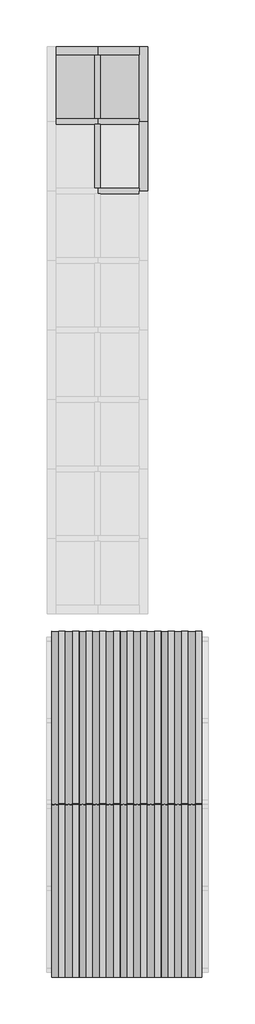
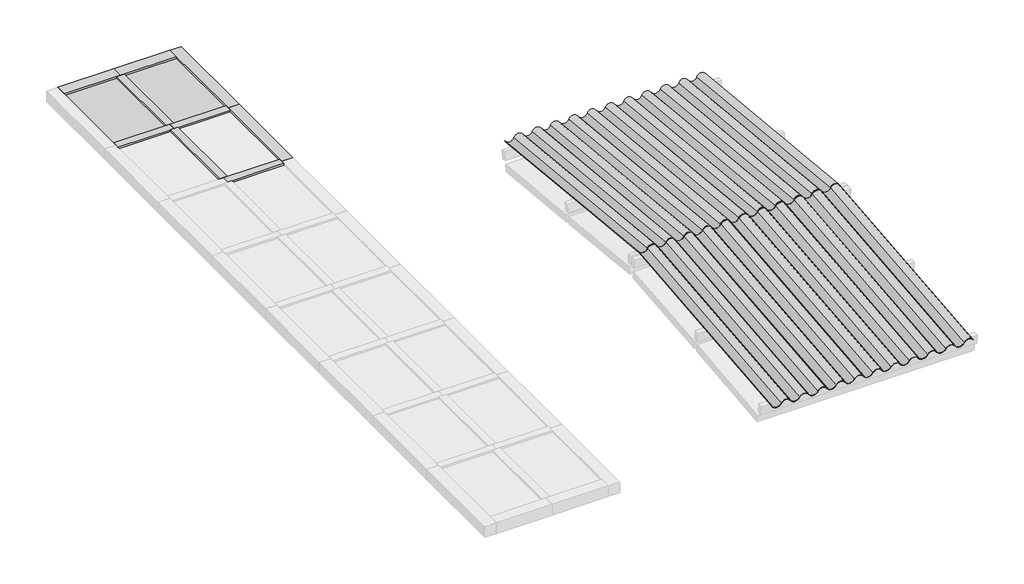
# One storey, part 2 of 2: 22 beams, 9 members, 2 plates.
"""IFC4 building model written with IfcOpenShell, lengths in millimetres."""

import ifcopenshell
import ifcopenshell.guid

model = None  # the IFC model being written
_history = None  # IfcOwnerHistory: only IFC2X3 demands one
_inside = {}  # id of a spatial element -> (the spatial element, [elements in it])
_under = {}  # id of a project, library or spatial element -> (it, [spatial elements below it])
_declared = {}  # id of a project -> (the project, [libraries it declares])
_typed = {}  # id of a type object -> (the type object, [elements of that type])
_made_of = {}  # id of a material, layer set ... -> (it, [elements and type objects made of it])


def new_model(schema):
    """Start an empty IFC model of exactly this schema.

    Asked for "IFC4X3", IfcOpenShell would pick the latest addendum, in which some entities
    have other attributes; the version numbers below select the first issue.
    IFC2X3 requires an IfcOwnerHistory on every rooted entity: one is made here for all.
    """
    global model, _history
    if schema == "IFC4X3":
        model = ifcopenshell.file(schema_version=(4, 3, 0, 0))
    else:
        model = ifcopenshell.file(schema=schema)
    _inside.clear()
    _under.clear()
    _declared.clear()
    _typed.clear()
    _made_of.clear()
    _history = None
    if model.schema == "IFC2X3":
        org = make("IfcOrganization", Name="unknown")
        user = make(
            "IfcPersonAndOrganization",
            ThePerson=make("IfcPerson", FamilyName="unknown"),
            TheOrganization=org,
        )
        app = make(
            "IfcApplication",
            ApplicationDeveloper=org,
            Version="unknown",
            ApplicationFullName="unknown",
            ApplicationIdentifier="unknown",
        )
        _history = make(
            "IfcOwnerHistory",
            OwningUser=user,
            OwningApplication=app,
            ChangeAction="ADDED",
            CreationDate=0,
        )
    return model


def make(cls, **values):
    """One entity of the class cls with the attributes given. An attribute that is None is left unset."""
    return model.create_entity(
        cls, **{name: value for name, value in values.items() if value is not None}
    )


def rooted(cls, **values):
    """An entity with a GlobalId (a new one), such as an element, a storey or a relation."""
    return make(cls, GlobalId=ifcopenshell.guid.new(), OwnerHistory=_history, **values)


def si_unit(unit_type, name, prefix=None):
    """IfcSIUnit, for example si_unit("LENGTHUNIT", "METRE", prefix="MILLI")."""
    return make("IfcSIUnit", UnitType=unit_type, Prefix=prefix, Name=name)


def assignment(units):
    """IfcUnitAssignment: the units of a project."""
    return None if units is None else make("IfcUnitAssignment", Units=units)


def point(xyz):
    """IfcCartesianPoint."""
    return None if xyz is None else make("IfcCartesianPoint", Coordinates=xyz)


def direction(xyz):
    """IfcDirection."""
    return None if xyz is None else make("IfcDirection", DirectionRatios=xyz)


def frame(location, z_axis=None, x_axis=None):
    """IfcAxis2Placement3D, a coordinate frame: its origin and axes. An axis left out is left unset."""
    return make(
        "IfcAxis2Placement3D",
        Location=point(location),
        Axis=direction(z_axis),
        RefDirection=direction(x_axis),
    )


def frame_2d(location, x_axis=None):
    """IfcAxis2Placement2D, a coordinate frame in the plane: its origin and x axis."""
    return make(
        "IfcAxis2Placement2D", Location=point(location), RefDirection=direction(x_axis)
    )


def origin():
    """The frame at (0, 0, 0) with its axes left unset."""
    return frame((0.0, 0.0, 0.0))


def origin_with_axes():
    """The frame at (0, 0, 0) with the z axis (0, 0, 1) and the x axis (1, 0, 0) written out."""
    return frame((0.0, 0.0, 0.0), z_axis=(0.0, 0.0, 1.0), x_axis=(1.0, 0.0, 0.0))


def place(relative_to, where):
    """IfcLocalPlacement: puts the frame where relative to a parent placement (None: the world)."""
    return make(
        "IfcLocalPlacement", PlacementRelTo=relative_to, RelativePlacement=where
    )


def context(
    kind, dimensions, precision=None, world=None, true_north=None, identifier=None
):
    """IfcGeometricRepresentationContext, for example the 3D "Model" context."""
    return make(
        "IfcGeometricRepresentationContext",
        ContextIdentifier=identifier,
        ContextType=kind,
        CoordinateSpaceDimension=dimensions,
        Precision=precision,
        WorldCoordinateSystem=world,
        TrueNorth=true_north,
    )


def project(units=None, contexts=None):
    """IfcProject with its units and contexts."""
    return rooted(
        "IfcProject",
        Name="project",
        RepresentationContexts=contexts,
        UnitsInContext=assignment(units),
    )


def spatial(cls, under=None, at=None, **own):
    """A site, building, storey or space (cls), placed at a placement, below another one or the project."""
    s = rooted(cls, ObjectPlacement=at, **own)
    if under is not None:
        _under.setdefault(under.id(), (under, []))[1].append(s)
    return s


def polyline(points):
    """IfcPolyline through the points."""
    return make("IfcPolyline", Points=[point(p) for p in points])


def circle_curve(where, radius):
    """IfcCircle in the frame where."""
    return make("IfcCircle", Position=where, Radius=radius)


def trimmed(basis, trim1, trim2, sense, master):
    """IfcTrimmedCurve: the piece of a basis curve between two trims."""
    return make(
        "IfcTrimmedCurve",
        BasisCurve=basis,
        Trim1=trim1,
        Trim2=trim2,
        SenseAgreement=sense,
        MasterRepresentation=master,
    )


def segment(curve, same_sense, transition):
    """IfcCompositeCurveSegment."""
    return make(
        "IfcCompositeCurveSegment",
        Transition=transition,
        SameSense=same_sense,
        ParentCurve=curve,
    )


def composite_curve(segments, self_intersect=None):
    """IfcCompositeCurve: segments joined end to end."""
    return make("IfcCompositeCurve", Segments=segments, SelfIntersect=self_intersect)


def outline(outer, holes=None, kind="AREA"):
    """IfcArbitraryClosedProfileDef: a profile drawn as a closed curve; with holes, ...WithVoids."""
    if holes is None:
        return make("IfcArbitraryClosedProfileDef", ProfileType=kind, OuterCurve=outer)
    return make(
        "IfcArbitraryProfileDefWithVoids",
        ProfileType=kind,
        OuterCurve=outer,
        InnerCurves=holes,
    )


def extrude(swept, where, along, depth):
    """IfcExtrudedAreaSolid: the profile swept, set in the frame where, extruded along a direction by depth."""
    return make(
        "IfcExtrudedAreaSolid",
        SweptArea=swept,
        Position=where,
        ExtrudedDirection=direction(along),
        Depth=depth,
    )


def shape(context_of_items, identifier, shape_type, items):
    """IfcShapeRepresentation: the items that make up one representation, for example the "Body"."""
    return make(
        "IfcShapeRepresentation",
        ContextOfItems=context_of_items,
        RepresentationIdentifier=identifier,
        RepresentationType=shape_type,
        Items=items,
    )


def source(mapping_origin, context_of_items, identifier, shape_type, items):
    """IfcRepresentationMap: a shape defined once, which mapped items show again and again."""
    return make(
        "IfcRepresentationMap",
        MappingOrigin=mapping_origin,
        MappedRepresentation=shape(context_of_items, identifier, shape_type, items),
    )


def transform(
    local_origin,
    x_axis=None,
    y_axis=None,
    z_axis=None,
    scale=None,
    scale2=None,
    scale3=None,
    uniform=True,
):
    """IfcCartesianTransformationOperator3D, or its non-uniform kind. x_axis, y_axis, z_axis: its Axis1, 2, 3."""
    if uniform:
        return make(
            "IfcCartesianTransformationOperator3D",
            Axis1=direction(x_axis),
            Axis2=direction(y_axis),
            LocalOrigin=point(local_origin),
            Scale=scale,
            Axis3=direction(z_axis),
        )
    return make(
        "IfcCartesianTransformationOperator3DnonUniform",
        Axis1=direction(x_axis),
        Axis2=direction(y_axis),
        LocalOrigin=point(local_origin),
        Scale=scale,
        Axis3=direction(z_axis),
        Scale2=scale2,
        Scale3=scale3,
    )


def mapped(mapping_source, mapping_target):
    """IfcMappedItem: shows the shape of a source again, moved by a transform."""
    return make(
        "IfcMappedItem", MappingSource=mapping_source, MappingTarget=mapping_target
    )


def made_of(thing, what):
    """Note that an element or type object is made of a material, layer set ...; save() writes the relation."""
    if what is not None:
        _made_of.setdefault(what.id(), (what, []))[1].append(thing)
    return thing


def element(
    cls,
    number,
    at=None,
    inside=None,
    cuts=None,
    type_object=None,
    material=None,
    context=None,
    identifier="Body",
    shape_type=None,
    held_by="IfcProductDefinitionShape",
    body=None,
    shapes=None,
    **own,
):
    """One element of the class cls, such as IfcWall. Its Tag is "e" and its number.

    at: its placement. inside: the storey or other place that contains it. cuts: it is an
    opening in that element (IfcRelVoidsElement). A single representation is given by context,
    identifier, shape_type and body (its items); several are given by shapes. held_by: the class
    of the entity that holds the representations. save() writes the other relations.
    """
    e = rooted(cls, Tag="e%d" % number, ObjectPlacement=at, **own)
    if body is not None:
        shapes = [shape(context, identifier, shape_type, body)]
    if shapes is not None:
        e.Representation = make(held_by, Representations=shapes)
    if inside is not None:
        _inside.setdefault(inside.id(), (inside, []))[1].append(e)
    if cuts is not None:
        rooted(
            "IfcRelVoidsElement", RelatingBuildingElement=cuts, RelatedOpeningElement=e
        )
    if type_object is not None:
        _typed.setdefault(type_object.id(), (type_object, []))[1].append(e)
    return made_of(e, material)


def aggregate(whole, parts):
    """IfcRelAggregates: a whole, such as a stair, and the parts it consists of."""
    return rooted("IfcRelAggregates", RelatingObject=whole, RelatedObjects=parts)


def save(model, path):
    """Write the relations noted so far, then the file.

    IfcRelAggregates (storeys below a building ...), IfcRelContainedInSpatialStructure (elements
    in a storey), IfcRelDefinesByType, IfcRelAssociatesMaterial and IfcRelDeclares: one each for
    every whole, place, type object, material and project.
    """
    for whole, parts in _under.values():
        aggregate(whole, parts)
    for where, things in _inside.values():
        rooted(
            "IfcRelContainedInSpatialStructure",
            RelatedElements=things,
            RelatingStructure=where,
        )
    for kind, things in _typed.values():
        rooted("IfcRelDefinesByType", RelatedObjects=things, RelatingType=kind)
    for what, things in _made_of.values():
        rooted("IfcRelAssociatesMaterial", RelatedObjects=things, RelatingMaterial=what)
    for by, libraries in _declared.values():
        rooted("IfcRelDeclares", RelatingContext=by, RelatedDefinitions=libraries)
    model.write(path)


def montante_retangular_d0ec09bd(model_context):
    return source(origin(), model_context, "Body", "SweptSolid", [
        extrude(outline(polyline([(50.0, 75.0), (50.0, -75.0), (-50.0, -75.0), (-50.0, 75.0), (50.0, 75.0)])), frame((0.0, 0.0, -1143.7500002), z_axis=(0.0, 0.0, 1.0), x_axis=(1.0, 0.0, 0.0)), (0.0, 0.0, 1.0), 1143.7500002),
    ])


def montante_retangular_ab766952(model_context):
    return source(origin(), model_context, "Body", "SweptSolid", [
        extrude(outline(polyline([(50.0, 75.0), (50.0, -75.0), (-50.0, -75.0), (-50.0, 75.0), (50.0, 75.0)])), frame((0.0, 0.0, -750.0), z_axis=(0.0, 0.0, 1.0), x_axis=(1.0, 0.0, 0.0)), (0.0, 0.0, 1.0), 750.0),
    ])


def montante_retangular_cc_150_x_150_mm_106b3bff(model_context):
    return source(origin(), model_context, "Body", "SweptSolid", [
        extrude(outline(polyline([(0.0, 75.0), (0.0, -75.0), (-150.0, -75.0), (-150.0, 75.0), (0.0, 75.0)])), frame((0.0, 0.0, -1343.7500002), z_axis=(0.0, 0.0, 1.0), x_axis=(1.0, 0.0, 0.0)), (0.0, 0.0, 1.0), 1343.7500002),
    ])


def montante_retangular_cc_150_x_150_mm_9af7129c(model_context):
    return source(origin(), model_context, "Body", "SweptSolid", [
        extrude(outline(polyline([(0.0, 75.0), (0.0, -75.0), (-150.0, -75.0), (-150.0, 75.0), (0.0, 75.0)])), frame((0.0, 0.0, -750.0), z_axis=(0.0, 0.0, 1.0), x_axis=(1.0, 0.0, 0.0)), (0.0, 0.0, 1.0), 750.0),
    ])


def montante_retangular_cc_150_x_150_mm_95775847(model_context):
    return source(origin(), model_context, "Body", "SweptSolid", [
        extrude(outline(polyline([(0.0, 75.0), (0.0, -75.0), (-150.0, -75.0), (-150.0, 75.0), (0.0, 75.0)])), frame((0.0, 0.0, -1243.7499999), z_axis=(0.0, 0.0, 1.0), x_axis=(1.0, 0.0, 0.0)), (0.0, 0.0, 1.0), 1243.7499999),
    ])


def painel_do_sistema_e7d0d29a(model_context):
    return source(origin(), model_context, "Body", "SweptSolid", [
        extrude(outline(polyline([(571.8750001, -49.5), (-571.8750001, -49.5), (-571.8750001, -24.5), (571.8750001, -24.5), (571.8750001, -49.5)])), origin_with_axes(), (0.0, 0.0, 1.0), 700.0),
    ])


model = new_model("IFC4")

# Units and contexts
model_context = context("Model", 3, world=origin())
ifc_project = project(units=[si_unit("LENGTHUNIT", "METRE", prefix="MILLI")], contexts=[model_context])

# Site, building, storey
site = spatial("IfcSite", under=ifc_project)
building = spatial("IfcBuilding", under=site)
storey = spatial("IfcBuildingStorey", under=building, Name="COB. CAIXA D'ÁGUA", Elevation=8750.0)

# Beams
placement = place(None, origin())
element("IfcBeam", 1, ObjectType="Telha Ondulada : Fibrocimento", at=placement, inside=storey, context=model_context, shape_type="SweptSolid", body=[
    extrude(outline(composite_curve([segment(trimmed(circle_curve(frame_2d((-58.7002978, -53.2060539)), 66.7939461), [point((-29.3501489, 6.7939461))], [point((-29.3501489, -113.2060539))], False, "CARTESIAN"), True, "CONTINUOUS"), segment(polyline([(-29.3501489, -113.2060539), (-31.5472154, -108.7146289)]), True, "CONTINUOUS"), segment(trimmed(circle_curve(frame_2d((-58.7002978, -53.2060539)), 61.7939461), [point((-31.5472154, -108.7146289))], [point((-31.5472154, 2.3025211))], True, "CARTESIAN"), True, "CONTINUOUS"), segment(trimmed(circle_curve(frame_2d((0.0, 66.7939461)), 71.7939461), [point((-31.5472154, 2.3025211))], [point((-31.5472154, 131.2853711))], False, "CARTESIAN"), True, "CONTINUOUS"), segment(polyline([(-31.5472154, 131.2853711), (-29.3501489, 126.7939461)]), True, "CONTINUOUS"), segment(trimmed(circle_curve(frame_2d((0.0, 66.7939461)), 66.7939461), [point((-29.3501489, 126.7939461))], [point((-29.3501489, 6.7939461))], True, "CARTESIAN"), True, "CONTINUOUS")], self_intersect=False)), frame((199.6156257, -4662.1614585, 9090.9296777), z_axis=(0.0, -0.9950371902099893, 0.09950371902099821), x_axis=(0.0, 0.09950371902099821, 0.9950371902099893)), (0.0, 0.0, 1.0), 3103.677649),
])
element("IfcBeam", 2, ObjectType="Telha Ondulada : Fibrocimento", at=placement, inside=storey, context=model_context, shape_type="SweptSolid", body=[
    extrude(outline(composite_curve([segment(trimmed(circle_curve(frame_2d((-58.7002978, -53.2060539)), 66.7939461), [point((-29.3501489, 6.7939461))], [point((-29.3501489, -113.2060539))], False, "CARTESIAN"), True, "CONTINUOUS"), segment(polyline([(-29.3501489, -113.2060539), (-31.5472154, -108.7146289)]), True, "CONTINUOUS"), segment(trimmed(circle_curve(frame_2d((-58.7002978, -53.2060539)), 61.7939461), [point((-31.5472154, -108.7146289))], [point((-31.5472154, 2.3025211))], True, "CARTESIAN"), True, "CONTINUOUS"), segment(trimmed(circle_curve(frame_2d((0.0, 66.7939461)), 71.7939461), [point((-31.5472154, 2.3025211))], [point((-31.5472154, 131.2853711))], False, "CARTESIAN"), True, "CONTINUOUS"), segment(polyline([(-31.5472154, 131.2853711), (-29.3501489, 126.7939461)]), True, "CONTINUOUS"), segment(trimmed(circle_curve(frame_2d((0.0, 66.7939461)), 66.7939461), [point((-29.3501489, 126.7939461))], [point((-29.3501489, 6.7939461))], True, "CARTESIAN"), True, "CONTINUOUS")], self_intersect=False)), frame((444.1156257, -4662.1614585, 9090.9296777), z_axis=(0.0, -0.9950371902099893, 0.09950371902099821), x_axis=(0.0, 0.09950371902099821, 0.9950371902099893)), (0.0, 0.0, 1.0), 3103.677649),
])
element("IfcBeam", 3, ObjectType="Telha Ondulada : Fibrocimento", at=placement, inside=storey, context=model_context, shape_type="SweptSolid", body=[
    extrude(outline(composite_curve([segment(trimmed(circle_curve(frame_2d((-58.7002978, -53.2060539)), 66.7939461), [point((-29.3501489, 6.7939461))], [point((-29.3501489, -113.2060539))], False, "CARTESIAN"), True, "CONTINUOUS"), segment(polyline([(-29.3501489, -113.2060539), (-31.5472154, -108.7146289)]), True, "CONTINUOUS"), segment(trimmed(circle_curve(frame_2d((-58.7002978, -53.2060539)), 61.7939461), [point((-31.5472154, -108.7146289))], [point((-31.5472154, 2.3025211))], True, "CARTESIAN"), True, "CONTINUOUS"), segment(trimmed(circle_curve(frame_2d((0.0, 66.7939461)), 71.7939461), [point((-31.5472154, 2.3025211))], [point((-31.5472154, 131.2853711))], False, "CARTESIAN"), True, "CONTINUOUS"), segment(polyline([(-31.5472154, 131.2853711), (-29.3501489, 126.7939461)]), True, "CONTINUOUS"), segment(trimmed(circle_curve(frame_2d((0.0, 66.7939461)), 66.7939461), [point((-29.3501489, 126.7939461))], [point((-29.3501489, 6.7939461))], True, "CARTESIAN"), True, "CONTINUOUS")], self_intersect=False)), frame((688.6156257, -4662.1614585, 9090.9296777), z_axis=(0.0, -0.9950371902099893, 0.09950371902099821), x_axis=(0.0, 0.09950371902099821, 0.9950371902099893)), (0.0, 0.0, 1.0), 3103.677649),
])
element("IfcBeam", 4, ObjectType="Telha Ondulada : Fibrocimento", at=placement, inside=storey, context=model_context, shape_type="SweptSolid", body=[
    extrude(outline(composite_curve([segment(trimmed(circle_curve(frame_2d((-58.7002978, -53.2060539)), 66.7939461), [point((-29.3501489, 6.7939461))], [point((-29.3501489, -113.2060539))], False, "CARTESIAN"), True, "CONTINUOUS"), segment(polyline([(-29.3501489, -113.2060539), (-31.5472154, -108.7146289)]), True, "CONTINUOUS"), segment(trimmed(circle_curve(frame_2d((-58.7002978, -53.2060539)), 61.7939461), [point((-31.5472154, -108.7146289))], [point((-31.5472154, 2.3025211))], True, "CARTESIAN"), True, "CONTINUOUS"), segment(trimmed(circle_curve(frame_2d((0.0, 66.7939461)), 71.7939461), [point((-31.5472154, 2.3025211))], [point((-31.5472154, 131.2853711))], False, "CARTESIAN"), True, "CONTINUOUS"), segment(polyline([(-31.5472154, 131.2853711), (-29.3501489, 126.7939461)]), True, "CONTINUOUS"), segment(trimmed(circle_curve(frame_2d((0.0, 66.7939461)), 66.7939461), [point((-29.3501489, 126.7939461))], [point((-29.3501489, 6.7939461))], True, "CARTESIAN"), True, "CONTINUOUS")], self_intersect=False)), frame((933.1156257, -4662.1614585, 9090.9296777), z_axis=(0.0, -0.9950371902099893, 0.09950371902099821), x_axis=(0.0, 0.09950371902099821, 0.9950371902099893)), (0.0, 0.0, 1.0), 3103.677649),
])
element("IfcBeam", 5, ObjectType="Telha Ondulada : Fibrocimento", at=placement, inside=storey, context=model_context, shape_type="SweptSolid", body=[
    extrude(outline(composite_curve([segment(trimmed(circle_curve(frame_2d((-58.7002978, -53.2060539)), 66.7939461), [point((-29.3501489, 6.7939461))], [point((-29.3501489, -113.2060539))], False, "CARTESIAN"), True, "CONTINUOUS"), segment(polyline([(-29.3501489, -113.2060539), (-31.5472154, -108.7146289)]), True, "CONTINUOUS"), segment(trimmed(circle_curve(frame_2d((-58.7002978, -53.2060539)), 61.7939461), [point((-31.5472154, -108.7146289))], [point((-31.5472154, 2.3025211))], True, "CARTESIAN"), True, "CONTINUOUS"), segment(trimmed(circle_curve(frame_2d((0.0, 66.7939461)), 71.7939461), [point((-31.5472154, 2.3025211))], [point((-31.5472154, 131.2853711))], False, "CARTESIAN"), True, "CONTINUOUS"), segment(polyline([(-31.5472154, 131.2853711), (-29.3501489, 126.7939461)]), True, "CONTINUOUS"), segment(trimmed(circle_curve(frame_2d((0.0, 66.7939461)), 66.7939461), [point((-29.3501489, 126.7939461))], [point((-29.3501489, 6.7939461))], True, "CARTESIAN"), True, "CONTINUOUS")], self_intersect=False)), frame((1177.6156257, -4662.1614585, 9090.9296777), z_axis=(0.0, -0.9950371902099893, 0.09950371902099821), x_axis=(0.0, 0.09950371902099821, 0.9950371902099893)), (0.0, 0.0, 1.0), 3103.677649),
])
element("IfcBeam", 6, ObjectType="Telha Ondulada : Fibrocimento", at=placement, inside=storey, context=model_context, shape_type="SweptSolid", body=[
    extrude(outline(composite_curve([segment(trimmed(circle_curve(frame_2d((-58.7002978, -53.2060539)), 66.7939461), [point((-29.3501489, 6.7939461))], [point((-29.3501489, -113.2060539))], False, "CARTESIAN"), True, "CONTINUOUS"), segment(polyline([(-29.3501489, -113.2060539), (-31.5472154, -108.7146289)]), True, "CONTINUOUS"), segment(trimmed(circle_curve(frame_2d((-58.7002978, -53.2060539)), 61.7939461), [point((-31.5472154, -108.7146289))], [point((-31.5472154, 2.3025211))], True, "CARTESIAN"), True, "CONTINUOUS"), segment(trimmed(circle_curve(frame_2d((0.0, 66.7939461)), 71.7939461), [point((-31.5472154, 2.3025211))], [point((-31.5472154, 131.2853711))], False, "CARTESIAN"), True, "CONTINUOUS"), segment(polyline([(-31.5472154, 131.2853711), (-29.3501489, 126.7939461)]), True, "CONTINUOUS"), segment(trimmed(circle_curve(frame_2d((0.0, 66.7939461)), 66.7939461), [point((-29.3501489, 126.7939461))], [point((-29.3501489, 6.7939461))], True, "CARTESIAN"), True, "CONTINUOUS")], self_intersect=False)), frame((1422.1156257, -4662.1614585, 9090.9296777), z_axis=(0.0, -0.9950371902099893, 0.09950371902099789), x_axis=(0.0, 0.09950371902099789, 0.9950371902099893)), (0.0, 0.0, 1.0), 3103.677649),
])
element("IfcBeam", 7, ObjectType="Telha Ondulada : Fibrocimento", at=placement, inside=storey, context=model_context, shape_type="SweptSolid", body=[
    extrude(outline(composite_curve([segment(trimmed(circle_curve(frame_2d((-58.7002978, -53.2060539)), 66.7939461), [point((-29.3501489, 6.7939461))], [point((-29.3501489, -113.2060539))], False, "CARTESIAN"), True, "CONTINUOUS"), segment(polyline([(-29.3501489, -113.2060539), (-31.5472154, -108.7146289)]), True, "CONTINUOUS"), segment(trimmed(circle_curve(frame_2d((-58.7002978, -53.2060539)), 61.7939461), [point((-31.5472154, -108.7146289))], [point((-31.5472154, 2.3025211))], True, "CARTESIAN"), True, "CONTINUOUS"), segment(trimmed(circle_curve(frame_2d((0.0, 66.7939461)), 71.7939461), [point((-31.5472154, 2.3025211))], [point((-31.5472154, 131.2853711))], False, "CARTESIAN"), True, "CONTINUOUS"), segment(polyline([(-31.5472154, 131.2853711), (-29.3501489, 126.7939461)]), True, "CONTINUOUS"), segment(trimmed(circle_curve(frame_2d((0.0, 66.7939461)), 66.7939461), [point((-29.3501489, 126.7939461))], [point((-29.3501489, 6.7939461))], True, "CARTESIAN"), True, "CONTINUOUS")], self_intersect=False)), frame((1666.6156257, -4662.1614585, 9090.9296777), z_axis=(0.0, -0.9950371902099893, 0.09950371902099789), x_axis=(0.0, 0.09950371902099789, 0.9950371902099893)), (0.0, 0.0, 1.0), 3103.677649),
])
element("IfcBeam", 8, ObjectType="Telha Ondulada : Fibrocimento", at=placement, inside=storey, context=model_context, shape_type="SweptSolid", body=[
    extrude(outline(composite_curve([segment(trimmed(circle_curve(frame_2d((-58.7002978, -53.2060539)), 66.7939461), [point((-29.3501489, 6.7939461))], [point((-29.3501489, -113.2060539))], False, "CARTESIAN"), True, "CONTINUOUS"), segment(polyline([(-29.3501489, -113.2060539), (-31.5472154, -108.7146289)]), True, "CONTINUOUS"), segment(trimmed(circle_curve(frame_2d((-58.7002978, -53.2060539)), 61.7939461), [point((-31.5472154, -108.7146289))], [point((-31.5472154, 2.3025211))], True, "CARTESIAN"), True, "CONTINUOUS"), segment(trimmed(circle_curve(frame_2d((0.0, 66.7939461)), 71.7939461), [point((-31.5472154, 2.3025211))], [point((-31.5472154, 131.2853711))], False, "CARTESIAN"), True, "CONTINUOUS"), segment(polyline([(-31.5472154, 131.2853711), (-29.3501489, 126.7939461)]), True, "CONTINUOUS"), segment(trimmed(circle_curve(frame_2d((0.0, 66.7939461)), 66.7939461), [point((-29.3501489, 126.7939461))], [point((-29.3501489, 6.7939461))], True, "CARTESIAN"), True, "CONTINUOUS")], self_intersect=False)), frame((1911.1156257, -4662.1614585, 9090.9296777), z_axis=(0.0, -0.9950371902099893, 0.09950371902099789), x_axis=(0.0, 0.09950371902099789, 0.9950371902099893)), (0.0, 0.0, 1.0), 3103.677649),
])
element("IfcBeam", 9, ObjectType="Telha Ondulada : Fibrocimento", at=placement, inside=storey, context=model_context, shape_type="SweptSolid", body=[
    extrude(outline(composite_curve([segment(trimmed(circle_curve(frame_2d((-58.7002978, -53.2060539)), 66.7939461), [point((-29.3501489, 6.7939461))], [point((-29.3501489, -113.2060539))], False, "CARTESIAN"), True, "CONTINUOUS"), segment(polyline([(-29.3501489, -113.2060539), (-31.5472154, -108.7146289)]), True, "CONTINUOUS"), segment(trimmed(circle_curve(frame_2d((-58.7002978, -53.2060539)), 61.7939461), [point((-31.5472154, -108.7146289))], [point((-31.5472154, 2.3025211))], True, "CARTESIAN"), True, "CONTINUOUS"), segment(trimmed(circle_curve(frame_2d((0.0, 66.7939461)), 71.7939461), [point((-31.5472154, 2.3025211))], [point((-31.5472154, 131.2853711))], False, "CARTESIAN"), True, "CONTINUOUS"), segment(polyline([(-31.5472154, 131.2853711), (-29.3501489, 126.7939461)]), True, "CONTINUOUS"), segment(trimmed(circle_curve(frame_2d((0.0, 66.7939461)), 66.7939461), [point((-29.3501489, 126.7939461))], [point((-29.3501489, 6.7939461))], True, "CARTESIAN"), True, "CONTINUOUS")], self_intersect=False)), frame((2155.6156257, -4662.1614585, 9090.9296777), z_axis=(0.0, -0.9950371902099893, 0.09950371902099789), x_axis=(0.0, 0.09950371902099789, 0.9950371902099893)), (0.0, 0.0, 1.0), 3103.677649),
])
element("IfcBeam", 10, ObjectType="Telha Ondulada : Fibrocimento", at=placement, inside=storey, context=model_context, shape_type="SweptSolid", body=[
    extrude(outline(composite_curve([segment(trimmed(circle_curve(frame_2d((-58.7002978, -53.2060539)), 66.7939461), [point((-29.3501489, 6.7939461))], [point((-29.3501489, -113.2060539))], False, "CARTESIAN"), True, "CONTINUOUS"), segment(polyline([(-29.3501489, -113.2060539), (-31.5472154, -108.7146289)]), True, "CONTINUOUS"), segment(trimmed(circle_curve(frame_2d((-58.7002978, -53.2060539)), 61.7939461), [point((-31.5472154, -108.7146289))], [point((-31.5472154, 2.3025211))], True, "CARTESIAN"), True, "CONTINUOUS"), segment(trimmed(circle_curve(frame_2d((0.0, 66.7939461)), 71.7939461), [point((-31.5472154, 2.3025211))], [point((-31.5472154, 131.2853711))], False, "CARTESIAN"), True, "CONTINUOUS"), segment(polyline([(-31.5472154, 131.2853711), (-29.3501489, 126.7939461)]), True, "CONTINUOUS"), segment(trimmed(circle_curve(frame_2d((0.0, 66.7939461)), 66.7939461), [point((-29.3501489, 126.7939461))], [point((-29.3501489, 6.7939461))], True, "CARTESIAN"), True, "CONTINUOUS")], self_intersect=False)), frame((2400.1156257, -4662.1614585, 9090.9296777), z_axis=(0.0, -0.9950371902099893, 0.09950371902099789), x_axis=(0.0, 0.09950371902099789, 0.9950371902099893)), (0.0, 0.0, 1.0), 3103.677649),
])
element("IfcBeam", 11, ObjectType="Telha Ondulada : Fibrocimento", at=placement, inside=storey, context=model_context, shape_type="SweptSolid", body=[
    extrude(outline(composite_curve([segment(trimmed(circle_curve(frame_2d((-58.7002978, -53.2060539)), 66.7939461), [point((-29.3501489, 6.7939461))], [point((-29.3501489, -113.2060539))], False, "CARTESIAN"), True, "CONTINUOUS"), segment(polyline([(-29.3501489, -113.2060539), (-31.5472154, -108.7146289)]), True, "CONTINUOUS"), segment(trimmed(circle_curve(frame_2d((-58.7002978, -53.2060539)), 61.7939461), [point((-31.5472154, -108.7146289))], [point((-31.5472154, 2.3025211))], True, "CARTESIAN"), True, "CONTINUOUS"), segment(trimmed(circle_curve(frame_2d((0.0, 66.7939461)), 71.7939461), [point((-31.5472154, 2.3025211))], [point((-31.5472154, 131.2853711))], False, "CARTESIAN"), True, "CONTINUOUS"), segment(polyline([(-31.5472154, 131.2853711), (-29.3501489, 126.7939461)]), True, "CONTINUOUS"), segment(trimmed(circle_curve(frame_2d((0.0, 66.7939461)), 66.7939461), [point((-29.3501489, 126.7939461))], [point((-29.3501489, 6.7939461))], True, "CARTESIAN"), True, "CONTINUOUS")], self_intersect=False)), frame((2644.6156257, -4662.1614585, 9090.9296777), z_axis=(0.0, -0.9950371902099893, 0.09950371902099789), x_axis=(0.0, 0.09950371902099789, 0.9950371902099893)), (0.0, 0.0, 1.0), 3103.677649),
])
element("IfcBeam", 12, ObjectType="Telha Ondulada : Fibrocimento", at=placement, inside=storey, context=model_context, shape_type="SweptSolid", body=[
    extrude(outline(composite_curve([segment(trimmed(circle_curve(frame_2d((0.0, 66.7939461)), 66.7939461), [point((29.3501489, 6.7939461))], [point((29.3501489, 126.7939461))], True, "CARTESIAN"), True, "CONTINUOUS"), segment(polyline([(29.3501489, 126.7939461), (31.5472154, 131.2853711)]), True, "CONTINUOUS"), segment(trimmed(circle_curve(frame_2d((0.0, 66.7939461)), 71.7939461), [point((31.5472154, 131.2853711))], [point((31.5472154, 2.3025211))], False, "CARTESIAN"), True, "CONTINUOUS"), segment(trimmed(circle_curve(frame_2d((58.7002978, -53.2060539)), 61.7939461), [point((31.5472154, 2.3025211))], [point((31.5472154, -108.7146289))], True, "CARTESIAN"), True, "CONTINUOUS"), segment(polyline([(31.5472154, -108.7146289), (29.3501489, -113.2060539)]), True, "CONTINUOUS"), segment(trimmed(circle_curve(frame_2d((58.7002978, -53.2060539)), 66.7939461), [point((29.3501489, -113.2060539))], [point((29.3501489, 6.7939461))], False, "CARTESIAN"), True, "CONTINUOUS")], self_intersect=False)), frame((199.6156257, -10856.9785109, 9090.7496777), z_axis=(0.0, 0.9950371902099894, 0.09950371902099744), x_axis=(0.0, 0.09950371902099744, -0.9950371902099894)), (0.0, 0.0, 1.0), 3103.677649),
])
element("IfcBeam", 13, ObjectType="Telha Ondulada : Fibrocimento", at=placement, inside=storey, context=model_context, shape_type="SweptSolid", body=[
    extrude(outline(composite_curve([segment(trimmed(circle_curve(frame_2d((0.0, 66.7939461)), 66.7939461), [point((29.3501489, 6.7939461))], [point((29.3501489, 126.7939461))], True, "CARTESIAN"), True, "CONTINUOUS"), segment(polyline([(29.3501489, 126.7939461), (31.5472154, 131.2853711)]), True, "CONTINUOUS"), segment(trimmed(circle_curve(frame_2d((0.0, 66.7939461)), 71.7939461), [point((31.5472154, 131.2853711))], [point((31.5472154, 2.3025211))], False, "CARTESIAN"), True, "CONTINUOUS"), segment(trimmed(circle_curve(frame_2d((58.7002978, -53.2060539)), 61.7939461), [point((31.5472154, 2.3025211))], [point((31.5472154, -108.7146289))], True, "CARTESIAN"), True, "CONTINUOUS"), segment(polyline([(31.5472154, -108.7146289), (29.3501489, -113.2060539)]), True, "CONTINUOUS"), segment(trimmed(circle_curve(frame_2d((58.7002978, -53.2060539)), 66.7939461), [point((29.3501489, -113.2060539))], [point((29.3501489, 6.7939461))], False, "CARTESIAN"), True, "CONTINUOUS")], self_intersect=False)), frame((444.1156257, -10856.9785109, 9090.7496777), z_axis=(0.0, 0.9950371902099894, 0.09950371902099744), x_axis=(0.0, 0.09950371902099744, -0.9950371902099894)), (0.0, 0.0, 1.0), 3103.677649),
])
element("IfcBeam", 14, ObjectType="Telha Ondulada : Fibrocimento", at=placement, inside=storey, context=model_context, shape_type="SweptSolid", body=[
    extrude(outline(composite_curve([segment(trimmed(circle_curve(frame_2d((0.0, 66.7939461)), 66.7939461), [point((29.3501489, 6.7939461))], [point((29.3501489, 126.7939461))], True, "CARTESIAN"), True, "CONTINUOUS"), segment(polyline([(29.3501489, 126.7939461), (31.5472154, 131.2853711)]), True, "CONTINUOUS"), segment(trimmed(circle_curve(frame_2d((0.0, 66.7939461)), 71.7939461), [point((31.5472154, 131.2853711))], [point((31.5472154, 2.3025211))], False, "CARTESIAN"), True, "CONTINUOUS"), segment(trimmed(circle_curve(frame_2d((58.7002978, -53.2060539)), 61.7939461), [point((31.5472154, 2.3025211))], [point((31.5472154, -108.7146289))], True, "CARTESIAN"), True, "CONTINUOUS"), segment(polyline([(31.5472154, -108.7146289), (29.3501489, -113.2060539)]), True, "CONTINUOUS"), segment(trimmed(circle_curve(frame_2d((58.7002978, -53.2060539)), 66.7939461), [point((29.3501489, -113.2060539))], [point((29.3501489, 6.7939461))], False, "CARTESIAN"), True, "CONTINUOUS")], self_intersect=False)), frame((688.6156257, -10856.9785109, 9090.7496777), z_axis=(0.0, 0.9950371902099894, 0.09950371902099744), x_axis=(0.0, 0.09950371902099744, -0.9950371902099894)), (0.0, 0.0, 1.0), 3103.677649),
])
element("IfcBeam", 15, ObjectType="Telha Ondulada : Fibrocimento", at=placement, inside=storey, context=model_context, shape_type="SweptSolid", body=[
    extrude(outline(composite_curve([segment(trimmed(circle_curve(frame_2d((0.0, 66.7939461)), 66.7939461), [point((29.3501489, 6.7939461))], [point((29.3501489, 126.7939461))], True, "CARTESIAN"), True, "CONTINUOUS"), segment(polyline([(29.3501489, 126.7939461), (31.5472154, 131.2853711)]), True, "CONTINUOUS"), segment(trimmed(circle_curve(frame_2d((0.0, 66.7939461)), 71.7939461), [point((31.5472154, 131.2853711))], [point((31.5472154, 2.3025211))], False, "CARTESIAN"), True, "CONTINUOUS"), segment(trimmed(circle_curve(frame_2d((58.7002978, -53.2060539)), 61.7939461), [point((31.5472154, 2.3025211))], [point((31.5472154, -108.7146289))], True, "CARTESIAN"), True, "CONTINUOUS"), segment(polyline([(31.5472154, -108.7146289), (29.3501489, -113.2060539)]), True, "CONTINUOUS"), segment(trimmed(circle_curve(frame_2d((58.7002978, -53.2060539)), 66.7939461), [point((29.3501489, -113.2060539))], [point((29.3501489, 6.7939461))], False, "CARTESIAN"), True, "CONTINUOUS")], self_intersect=False)), frame((933.1156257, -10856.9785109, 9090.7496777), z_axis=(0.0, 0.9950371902099894, 0.09950371902099744), x_axis=(0.0, 0.09950371902099744, -0.9950371902099894)), (0.0, 0.0, 1.0), 3103.677649),
])
element("IfcBeam", 16, ObjectType="Telha Ondulada : Fibrocimento", at=placement, inside=storey, context=model_context, shape_type="SweptSolid", body=[
    extrude(outline(composite_curve([segment(trimmed(circle_curve(frame_2d((0.0, 66.7939461)), 66.7939461), [point((29.3501489, 6.7939461))], [point((29.3501489, 126.7939461))], True, "CARTESIAN"), True, "CONTINUOUS"), segment(polyline([(29.3501489, 126.7939461), (31.5472154, 131.2853711)]), True, "CONTINUOUS"), segment(trimmed(circle_curve(frame_2d((0.0, 66.7939461)), 71.7939461), [point((31.5472154, 131.2853711))], [point((31.5472154, 2.3025211))], False, "CARTESIAN"), True, "CONTINUOUS"), segment(trimmed(circle_curve(frame_2d((58.7002978, -53.2060539)), 61.7939461), [point((31.5472154, 2.3025211))], [point((31.5472154, -108.7146289))], True, "CARTESIAN"), True, "CONTINUOUS"), segment(polyline([(31.5472154, -108.7146289), (29.3501489, -113.2060539)]), True, "CONTINUOUS"), segment(trimmed(circle_curve(frame_2d((58.7002978, -53.2060539)), 66.7939461), [point((29.3501489, -113.2060539))], [point((29.3501489, 6.7939461))], False, "CARTESIAN"), True, "CONTINUOUS")], self_intersect=False)), frame((1177.6156257, -10856.9785109, 9090.7496777), z_axis=(0.0, 0.9950371902099894, 0.09950371902099744), x_axis=(0.0, 0.09950371902099744, -0.9950371902099894)), (0.0, 0.0, 1.0), 3103.677649),
])
element("IfcBeam", 17, ObjectType="Telha Ondulada : Fibrocimento", at=placement, inside=storey, context=model_context, shape_type="SweptSolid", body=[
    extrude(outline(composite_curve([segment(trimmed(circle_curve(frame_2d((0.0, 66.7939461)), 66.7939461), [point((29.3501489, 6.7939461))], [point((29.3501489, 126.7939461))], True, "CARTESIAN"), True, "CONTINUOUS"), segment(polyline([(29.3501489, 126.7939461), (31.5472154, 131.2853711)]), True, "CONTINUOUS"), segment(trimmed(circle_curve(frame_2d((0.0, 66.7939461)), 71.7939461), [point((31.5472154, 131.2853711))], [point((31.5472154, 2.3025211))], False, "CARTESIAN"), True, "CONTINUOUS"), segment(trimmed(circle_curve(frame_2d((58.7002978, -53.2060539)), 61.7939461), [point((31.5472154, 2.3025211))], [point((31.5472154, -108.7146289))], True, "CARTESIAN"), True, "CONTINUOUS"), segment(polyline([(31.5472154, -108.7146289), (29.3501489, -113.2060539)]), True, "CONTINUOUS"), segment(trimmed(circle_curve(frame_2d((58.7002978, -53.2060539)), 66.7939461), [point((29.3501489, -113.2060539))], [point((29.3501489, 6.7939461))], False, "CARTESIAN"), True, "CONTINUOUS")], self_intersect=False)), frame((1422.1156257, -10856.9785109, 9090.7496777), z_axis=(0.0, 0.9950371902099894, 0.09950371902099744), x_axis=(0.0, 0.09950371902099744, -0.9950371902099894)), (0.0, 0.0, 1.0), 3103.677649),
])
element("IfcBeam", 18, ObjectType="Telha Ondulada : Fibrocimento", at=placement, inside=storey, context=model_context, shape_type="SweptSolid", body=[
    extrude(outline(composite_curve([segment(trimmed(circle_curve(frame_2d((0.0, 66.7939461)), 66.7939461), [point((29.3501489, 6.7939461))], [point((29.3501489, 126.7939461))], True, "CARTESIAN"), True, "CONTINUOUS"), segment(polyline([(29.3501489, 126.7939461), (31.5472154, 131.2853711)]), True, "CONTINUOUS"), segment(trimmed(circle_curve(frame_2d((0.0, 66.7939461)), 71.7939461), [point((31.5472154, 131.2853711))], [point((31.5472154, 2.3025211))], False, "CARTESIAN"), True, "CONTINUOUS"), segment(trimmed(circle_curve(frame_2d((58.7002978, -53.2060539)), 61.7939461), [point((31.5472154, 2.3025211))], [point((31.5472154, -108.7146289))], True, "CARTESIAN"), True, "CONTINUOUS"), segment(polyline([(31.5472154, -108.7146289), (29.3501489, -113.2060539)]), True, "CONTINUOUS"), segment(trimmed(circle_curve(frame_2d((58.7002978, -53.2060539)), 66.7939461), [point((29.3501489, -113.2060539))], [point((29.3501489, 6.7939461))], False, "CARTESIAN"), True, "CONTINUOUS")], self_intersect=False)), frame((1666.6156257, -10856.9785109, 9090.7496777), z_axis=(0.0, 0.9950371902099894, 0.09950371902099744), x_axis=(0.0, 0.09950371902099744, -0.9950371902099894)), (0.0, 0.0, 1.0), 3103.677649),
])
element("IfcBeam", 19, ObjectType="Telha Ondulada : Fibrocimento", at=placement, inside=storey, context=model_context, shape_type="SweptSolid", body=[
    extrude(outline(composite_curve([segment(trimmed(circle_curve(frame_2d((0.0, 66.7939461)), 66.7939461), [point((29.3501489, 6.7939461))], [point((29.3501489, 126.7939461))], True, "CARTESIAN"), True, "CONTINUOUS"), segment(polyline([(29.3501489, 126.7939461), (31.5472154, 131.2853711)]), True, "CONTINUOUS"), segment(trimmed(circle_curve(frame_2d((0.0, 66.7939461)), 71.7939461), [point((31.5472154, 131.2853711))], [point((31.5472154, 2.3025211))], False, "CARTESIAN"), True, "CONTINUOUS"), segment(trimmed(circle_curve(frame_2d((58.7002978, -53.2060539)), 61.7939461), [point((31.5472154, 2.3025211))], [point((31.5472154, -108.7146289))], True, "CARTESIAN"), True, "CONTINUOUS"), segment(polyline([(31.5472154, -108.7146289), (29.3501489, -113.2060539)]), True, "CONTINUOUS"), segment(trimmed(circle_curve(frame_2d((58.7002978, -53.2060539)), 66.7939461), [point((29.3501489, -113.2060539))], [point((29.3501489, 6.7939461))], False, "CARTESIAN"), True, "CONTINUOUS")], self_intersect=False)), frame((1911.1156257, -10856.9785109, 9090.7496777), z_axis=(0.0, 0.9950371902099894, 0.09950371902099744), x_axis=(0.0, 0.09950371902099744, -0.9950371902099894)), (0.0, 0.0, 1.0), 3103.677649),
])
element("IfcBeam", 20, ObjectType="Telha Ondulada : Fibrocimento", at=placement, inside=storey, context=model_context, shape_type="SweptSolid", body=[
    extrude(outline(composite_curve([segment(trimmed(circle_curve(frame_2d((0.0, 66.7939461)), 66.7939461), [point((29.3501489, 6.7939461))], [point((29.3501489, 126.7939461))], True, "CARTESIAN"), True, "CONTINUOUS"), segment(polyline([(29.3501489, 126.7939461), (31.5472154, 131.2853711)]), True, "CONTINUOUS"), segment(trimmed(circle_curve(frame_2d((0.0, 66.7939461)), 71.7939461), [point((31.5472154, 131.2853711))], [point((31.5472154, 2.3025211))], False, "CARTESIAN"), True, "CONTINUOUS"), segment(trimmed(circle_curve(frame_2d((58.7002978, -53.2060539)), 61.7939461), [point((31.5472154, 2.3025211))], [point((31.5472154, -108.7146289))], True, "CARTESIAN"), True, "CONTINUOUS"), segment(polyline([(31.5472154, -108.7146289), (29.3501489, -113.2060539)]), True, "CONTINUOUS"), segment(trimmed(circle_curve(frame_2d((58.7002978, -53.2060539)), 66.7939461), [point((29.3501489, -113.2060539))], [point((29.3501489, 6.7939461))], False, "CARTESIAN"), True, "CONTINUOUS")], self_intersect=False)), frame((2155.6156257, -10856.9785109, 9090.7496777), z_axis=(0.0, 0.9950371902099894, 0.09950371902099744), x_axis=(0.0, 0.09950371902099744, -0.9950371902099894)), (0.0, 0.0, 1.0), 3103.677649),
])
element("IfcBeam", 21, ObjectType="Telha Ondulada : Fibrocimento", at=placement, inside=storey, context=model_context, shape_type="SweptSolid", body=[
    extrude(outline(composite_curve([segment(trimmed(circle_curve(frame_2d((0.0, 66.7939461)), 66.7939461), [point((29.3501489, 6.7939461))], [point((29.3501489, 126.7939461))], True, "CARTESIAN"), True, "CONTINUOUS"), segment(polyline([(29.3501489, 126.7939461), (31.5472154, 131.2853711)]), True, "CONTINUOUS"), segment(trimmed(circle_curve(frame_2d((0.0, 66.7939461)), 71.7939461), [point((31.5472154, 131.2853711))], [point((31.5472154, 2.3025211))], False, "CARTESIAN"), True, "CONTINUOUS"), segment(trimmed(circle_curve(frame_2d((58.7002978, -53.2060539)), 61.7939461), [point((31.5472154, 2.3025211))], [point((31.5472154, -108.7146289))], True, "CARTESIAN"), True, "CONTINUOUS"), segment(polyline([(31.5472154, -108.7146289), (29.3501489, -113.2060539)]), True, "CONTINUOUS"), segment(trimmed(circle_curve(frame_2d((58.7002978, -53.2060539)), 66.7939461), [point((29.3501489, -113.2060539))], [point((29.3501489, 6.7939461))], False, "CARTESIAN"), True, "CONTINUOUS")], self_intersect=False)), frame((2400.1156257, -10856.9785109, 9090.7496777), z_axis=(0.0, 0.9950371902099894, 0.09950371902099744), x_axis=(0.0, 0.09950371902099744, -0.9950371902099894)), (0.0, 0.0, 1.0), 3103.677649),
])
element("IfcBeam", 22, ObjectType="Telha Ondulada : Fibrocimento", at=placement, inside=storey, context=model_context, shape_type="SweptSolid", body=[
    extrude(outline(composite_curve([segment(trimmed(circle_curve(frame_2d((0.0, 66.7939461)), 66.7939461), [point((29.3501489, 6.7939461))], [point((29.3501489, 126.7939461))], True, "CARTESIAN"), True, "CONTINUOUS"), segment(polyline([(29.3501489, 126.7939461), (31.5472154, 131.2853711)]), True, "CONTINUOUS"), segment(trimmed(circle_curve(frame_2d((0.0, 66.7939461)), 71.7939461), [point((31.5472154, 131.2853711))], [point((31.5472154, 2.3025211))], False, "CARTESIAN"), True, "CONTINUOUS"), segment(trimmed(circle_curve(frame_2d((58.7002978, -53.2060539)), 61.7939461), [point((31.5472154, 2.3025211))], [point((31.5472154, -108.7146289))], True, "CARTESIAN"), True, "CONTINUOUS"), segment(polyline([(31.5472154, -108.7146289), (29.3501489, -113.2060539)]), True, "CONTINUOUS"), segment(trimmed(circle_curve(frame_2d((58.7002978, -53.2060539)), 66.7939461), [point((29.3501489, -113.2060539))], [point((29.3501489, 6.7939461))], False, "CARTESIAN"), True, "CONTINUOUS")], self_intersect=False)), frame((2644.6156257, -10856.9785109, 9090.7496777), z_axis=(0.0, 0.9950371902099894, 0.09950371902099744), x_axis=(0.0, 0.09950371902099744, -0.9950371902099894)), (0.0, 0.0, 1.0), 3103.677649),
])

# Members
montante_retangular_shape = montante_retangular_d0ec09bd(model_context)
element("IfcMember", 23, ObjectType="Montante retangular : CC_100 X 150  mm", at=placement, inside=storey, context=model_context, shape_type="MappedRepresentation", body=[
    mapped(montante_retangular_shape, transform((890.718693, 5654.4300153, 3365.0), x_axis=(1.0, 0.0, 0.0), y_axis=(0.0, 0.0, -1.0), z_axis=(0.0, 1.0, 0.0))),
])
element("IfcMember", 24, ObjectType="Montante retangular : CC_100 X 150  mm", at=placement, inside=storey, context=model_context, shape_type="MappedRepresentation", body=[
    mapped(montante_retangular_shape, transform((890.718693, 4410.6800151, 3365.0), x_axis=(1.0, 0.0, 0.0), y_axis=(0.0, 0.0, -1.0), z_axis=(0.0, 1.0, 0.0))),
])
montante_retangular_2_shape = montante_retangular_ab766952(model_context)
element("IfcMember", 25, ObjectType="Montante retangular : CC_100 X 150  mm", at=placement, inside=storey, context=model_context, shape_type="MappedRepresentation", body=[
    mapped(montante_retangular_2_shape, transform((1640.718693, 4460.6800151, 3365.0), x_axis=(0.0, -1.0, 0.0), y_axis=(0.0, 0.0, -1.0), z_axis=(1.0, 0.0, 0.0))),
])
element("IfcMember", 26, ObjectType="Montante retangular : CC_100 X 150  mm", at=placement, inside=storey, context=model_context, shape_type="MappedRepresentation", body=[
    mapped(montante_retangular_2_shape, transform((1640.718693, 3216.9300151, 3365.0), x_axis=(0.0, -1.0, 0.0), y_axis=(0.0, 0.0, -1.0), z_axis=(1.0, 0.0, 0.0))),
])
element("IfcMember", 27, ObjectType="Montante retangular : CC_100 X 150  mm", at=placement, inside=storey, context=model_context, shape_type="MappedRepresentation", body=[
    mapped(montante_retangular_2_shape, transform((890.718693, 4460.6800151, 3365.0), x_axis=(0.0, -1.0, 0.0), y_axis=(0.0, 0.0, -1.0), z_axis=(1.0, 0.0, 0.0))),
])
montante_retangular_cc_150_x_150_mm_shape = montante_retangular_cc_150_x_150_mm_106b3bff(model_context)
element("IfcMember", 28, ObjectType="Montante retangular : CC_150 X 150 mm", at=placement, inside=storey, context=model_context, shape_type="MappedRepresentation", body=[
    mapped(montante_retangular_cc_150_x_150_mm_shape, transform((1790.718693, 5804.4300153, 3365.0), x_axis=(1.0, 0.0, 0.0), y_axis=(0.0, 0.0, -1.0), z_axis=(0.0, 1.0, 0.0))),
])
montante_retangular_cc_150_x_150_mm_2_shape = montante_retangular_cc_150_x_150_mm_9af7129c(model_context)
element("IfcMember", 29, ObjectType="Montante retangular : CC_150 X 150 mm", at=placement, inside=storey, context=model_context, shape_type="MappedRepresentation", body=[
    mapped(montante_retangular_cc_150_x_150_mm_2_shape, transform((140.718693, 5804.4300153, 3365.0), x_axis=(0.0, 1.0, 0.0), y_axis=(0.0, 0.0, -1.0), z_axis=(-1.0, 0.0, 0.0))),
])
montante_retangular_cc_150_x_150_mm_3_shape = montante_retangular_cc_150_x_150_mm_95775847(model_context)
element("IfcMember", 30, ObjectType="Montante retangular : CC_150 X 150 mm", at=placement, inside=storey, context=model_context, shape_type="MappedRepresentation", body=[
    mapped(montante_retangular_cc_150_x_150_mm_3_shape, transform((1790.718693, 4460.6800151, 3365.0), x_axis=(1.0, 0.0, 0.0), y_axis=(0.0, 0.0, -1.0), z_axis=(0.0, 1.0, 0.0))),
])
element("IfcMember", 31, ObjectType="Montante retangular : CC_150 X 150 mm", at=placement, inside=storey, context=model_context, shape_type="MappedRepresentation", body=[
    mapped(montante_retangular_cc_150_x_150_mm_2_shape, transform((890.718693, 5804.4300153, 3365.0), x_axis=(0.0, 1.0, 0.0), y_axis=(0.0, 0.0, -1.0), z_axis=(-1.0, 0.0, 0.0))),
])

# Plates
painel_do_sistema_shape = painel_do_sistema_e7d0d29a(model_context)
element("IfcPlate", 32, ObjectType="Painel do sistema : Envidraçado", at=placement, inside=storey, context=model_context, shape_type="MappedRepresentation", body=[
    mapped(painel_do_sistema_shape, transform((140.718693, 5082.5550152, 3365.0), x_axis=(0.0, -1.0, 0.0), y_axis=(0.0, 0.0, -1.0), z_axis=(1.0, 0.0, 0.0))),
])
element("IfcPlate", 33, ObjectType="Painel do sistema : Envidraçado", at=placement, inside=storey, context=model_context, shape_type="MappedRepresentation", body=[
    mapped(painel_do_sistema_shape, transform((940.718693, 5082.5550152, 3365.0), x_axis=(0.0, -1.0, 0.0), y_axis=(0.0, 0.0, -1.0), z_axis=(1.0, 0.0, 0.0))),
])

save(model, "model.ifc")

# Revit data of these elements
# Type "Telha Ondulada : Fibrocimento"
#   Description = "TELHA ONDULADA FIBROCIMENTO"
#   Cost = 5
#   Length [instance default] = 1.524 m
#   b = 0.07 m
#   h = 0.16 m
#   Structural Material = .TELHA DE FIBROCIMENTO
#   Assembly Code = ""
# Type "Montante retangular : CC_100 X 150  mm"
#   built-in parameter 1007304 = 0.492126 (stored number, unit not read)
#   built-in parameter 1007301 = 0.164042 (stored number, unit not read)
#   built-in parameter 1007300 = 0.164042 (stored number, unit not read)
# Type "Montante retangular : CC_150 X 150 mm"
#   built-in parameter 1007304 = 0.492126 (stored number, unit not read)
#   built-in parameter 1007301 = 0.246063 (stored number, unit not read)
#   built-in parameter 1007300 = 0.246063 (stored number, unit not read)
# Type "Painel do sistema : Envidraçado"
#   Construction Type Id = "GSP4R"
#   Analytic Construction = "Vidraça única Pilkington 1/8 pol"
#   Visual Light Transmittance = 0.9
#   Solar Heat Gain Coefficient = 0.86
#   Heat Transfer Coefficient (U) = 6.7069 W/(m²·K)
# Elements 1, 2, 3, 4, 5, 6, 7, 8, 9, 10, 11, 12, 13, 14, 15, 16, 17, 18, 19, 20, 21, 22 (IfcBeam, "Telha Ondulada : Fibrocimento")
#   Phase Created = CC_PE
#   Materials on its faces: ".TELHA DE FIBROCIMENTO"
# Elements 23, 24, 25, 26, 27 (IfcMember, "Montante retangular : CC_100 X 150  mm")
#   Uso = "PERGOLADO PISCINA"
#   Phase Created = CC_AP
#   Materials on its faces: ".ALUMÍNIO"
# Elements 28, 29, 30, 31 (IfcMember, "Montante retangular : CC_150 X 150 mm")
#   Uso = "PERGOLADO PISCINA"
#   Phase Created = CC_AP
#   Materials on its faces: ".ALUMÍNIO"
# Elements 32, 33 (IfcPlate, "Painel do sistema : Envidraçado")
#   Uso = "PERGOLADO PISCINA"
#   Phase Created = CC_AP
#   Materials on its faces: ".VIDRO GENÉRICO"
# Materials
#   ".TELHA DE FIBROCIMENTO": class "CC_TELHADO", colour RGB 77 77 76, transparency 0, Description = "TELHA ONDULADA FIBROCIMENTO", Cost = 0
#   ".ALUMÍNIO": class "CC_METAIS", colour RGB 244 244 244, transparency 0, Description = "Material alumínio", Cost = 0
#   ".VIDRO GENÉRICO": class ".CC_VIDRO", colour RGB 0 128 192, transparency 0.9, Description = "Vidro comum", Cost = 0
